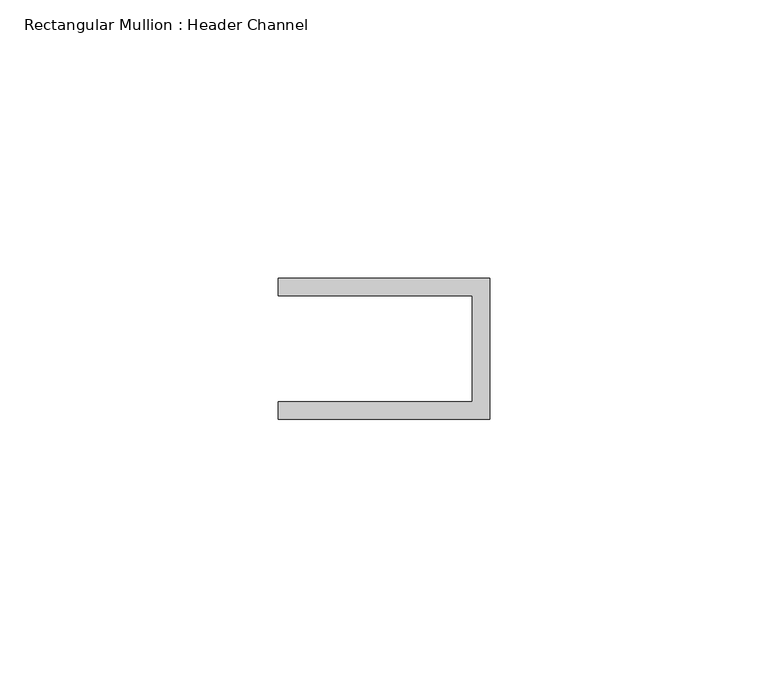
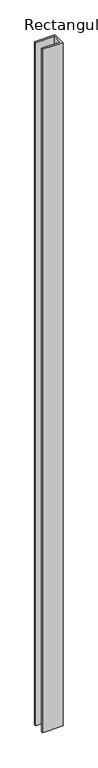
"""IFC4 building model written with IfcOpenShell, lengths in millimetres: member geometry, Rectangular Mullion : Header Channel."""

import ifcopenshell
import ifcopenshell.guid

model = None  # the IFC model being written
_history = None  # IfcOwnerHistory: only IFC2X3 demands one
_inside = {}  # id of a spatial element -> (the spatial element, [elements in it])
_under = {}  # id of a project, library or spatial element -> (it, [spatial elements below it])
_declared = {}  # id of a project -> (the project, [libraries it declares])
_typed = {}  # id of a type object -> (the type object, [elements of that type])
_made_of = {}  # id of a material, layer set ... -> (it, [elements and type objects made of it])


def new_model(schema):
    """Start an empty IFC model of exactly this schema.

    Asked for "IFC4X3", IfcOpenShell would pick the latest addendum, in which some entities
    have other attributes; the version numbers below select the first issue.
    IFC2X3 requires an IfcOwnerHistory on every rooted entity: one is made here for all.
    """
    global model, _history
    if schema == "IFC4X3":
        model = ifcopenshell.file(schema_version=(4, 3, 0, 0))
    else:
        model = ifcopenshell.file(schema=schema)
    _inside.clear()
    _under.clear()
    _declared.clear()
    _typed.clear()
    _made_of.clear()
    _history = None
    if model.schema == "IFC2X3":
        org = make("IfcOrganization", Name="unknown")
        user = make(
            "IfcPersonAndOrganization",
            ThePerson=make("IfcPerson", FamilyName="unknown"),
            TheOrganization=org,
        )
        app = make(
            "IfcApplication",
            ApplicationDeveloper=org,
            Version="unknown",
            ApplicationFullName="unknown",
            ApplicationIdentifier="unknown",
        )
        _history = make(
            "IfcOwnerHistory",
            OwningUser=user,
            OwningApplication=app,
            ChangeAction="ADDED",
            CreationDate=0,
        )
    return model


def make(cls, **values):
    """One entity of the class cls with the attributes given. An attribute that is None is left unset."""
    return model.create_entity(
        cls, **{name: value for name, value in values.items() if value is not None}
    )


def rooted(cls, **values):
    """An entity with a GlobalId (a new one), such as an element, a storey or a relation."""
    return make(cls, GlobalId=ifcopenshell.guid.new(), OwnerHistory=_history, **values)


def si_unit(unit_type, name, prefix=None):
    """IfcSIUnit, for example si_unit("LENGTHUNIT", "METRE", prefix="MILLI")."""
    return make("IfcSIUnit", UnitType=unit_type, Prefix=prefix, Name=name)


def assignment(units):
    """IfcUnitAssignment: the units of a project."""
    return None if units is None else make("IfcUnitAssignment", Units=units)


def point(xyz):
    """IfcCartesianPoint."""
    return None if xyz is None else make("IfcCartesianPoint", Coordinates=xyz)


def direction(xyz):
    """IfcDirection."""
    return None if xyz is None else make("IfcDirection", DirectionRatios=xyz)


def frame(location, z_axis=None, x_axis=None):
    """IfcAxis2Placement3D, a coordinate frame: its origin and axes. An axis left out is left unset."""
    return make(
        "IfcAxis2Placement3D",
        Location=point(location),
        Axis=direction(z_axis),
        RefDirection=direction(x_axis),
    )


def origin():
    """The frame at (0, 0, 0) with its axes left unset."""
    return frame((0.0, 0.0, 0.0))


def place(relative_to, where):
    """IfcLocalPlacement: puts the frame where relative to a parent placement (None: the world)."""
    return make(
        "IfcLocalPlacement", PlacementRelTo=relative_to, RelativePlacement=where
    )


def context(
    kind, dimensions, precision=None, world=None, true_north=None, identifier=None
):
    """IfcGeometricRepresentationContext, for example the 3D "Model" context."""
    return make(
        "IfcGeometricRepresentationContext",
        ContextIdentifier=identifier,
        ContextType=kind,
        CoordinateSpaceDimension=dimensions,
        Precision=precision,
        WorldCoordinateSystem=world,
        TrueNorth=true_north,
    )


def project(units=None, contexts=None):
    """IfcProject with its units and contexts."""
    return rooted(
        "IfcProject",
        Name="project",
        RepresentationContexts=contexts,
        UnitsInContext=assignment(units),
    )


def spatial(cls, under=None, at=None, **own):
    """A site, building, storey or space (cls), placed at a placement, below another one or the project."""
    s = rooted(cls, ObjectPlacement=at, **own)
    if under is not None:
        _under.setdefault(under.id(), (under, []))[1].append(s)
    return s


def polyline(points):
    """IfcPolyline through the points."""
    return make("IfcPolyline", Points=[point(p) for p in points])


def outline(outer, holes=None, kind="AREA"):
    """IfcArbitraryClosedProfileDef: a profile drawn as a closed curve; with holes, ...WithVoids."""
    if holes is None:
        return make("IfcArbitraryClosedProfileDef", ProfileType=kind, OuterCurve=outer)
    return make(
        "IfcArbitraryProfileDefWithVoids",
        ProfileType=kind,
        OuterCurve=outer,
        InnerCurves=holes,
    )


def extrude(swept, where, along, depth):
    """IfcExtrudedAreaSolid: the profile swept, set in the frame where, extruded along a direction by depth."""
    return make(
        "IfcExtrudedAreaSolid",
        SweptArea=swept,
        Position=where,
        ExtrudedDirection=direction(along),
        Depth=depth,
    )


def shape(context_of_items, identifier, shape_type, items):
    """IfcShapeRepresentation: the items that make up one representation, for example the "Body"."""
    return make(
        "IfcShapeRepresentation",
        ContextOfItems=context_of_items,
        RepresentationIdentifier=identifier,
        RepresentationType=shape_type,
        Items=items,
    )


def source(mapping_origin, context_of_items, identifier, shape_type, items):
    """IfcRepresentationMap: a shape defined once, which mapped items show again and again."""
    return make(
        "IfcRepresentationMap",
        MappingOrigin=mapping_origin,
        MappedRepresentation=shape(context_of_items, identifier, shape_type, items),
    )


def transform(
    local_origin,
    x_axis=None,
    y_axis=None,
    z_axis=None,
    scale=None,
    scale2=None,
    scale3=None,
    uniform=True,
):
    """IfcCartesianTransformationOperator3D, or its non-uniform kind. x_axis, y_axis, z_axis: its Axis1, 2, 3."""
    if uniform:
        return make(
            "IfcCartesianTransformationOperator3D",
            Axis1=direction(x_axis),
            Axis2=direction(y_axis),
            LocalOrigin=point(local_origin),
            Scale=scale,
            Axis3=direction(z_axis),
        )
    return make(
        "IfcCartesianTransformationOperator3DnonUniform",
        Axis1=direction(x_axis),
        Axis2=direction(y_axis),
        LocalOrigin=point(local_origin),
        Scale=scale,
        Axis3=direction(z_axis),
        Scale2=scale2,
        Scale3=scale3,
    )


def mapped(mapping_source, mapping_target):
    """IfcMappedItem: shows the shape of a source again, moved by a transform."""
    return make(
        "IfcMappedItem", MappingSource=mapping_source, MappingTarget=mapping_target
    )


def made_of(thing, what):
    """Note that an element or type object is made of a material, layer set ...; save() writes the relation."""
    if what is not None:
        _made_of.setdefault(what.id(), (what, []))[1].append(thing)
    return thing


def element(
    cls,
    number,
    at=None,
    inside=None,
    cuts=None,
    type_object=None,
    material=None,
    context=None,
    identifier="Body",
    shape_type=None,
    held_by="IfcProductDefinitionShape",
    body=None,
    shapes=None,
    **own,
):
    """One element of the class cls, such as IfcWall. Its Tag is "e" and its number.

    at: its placement. inside: the storey or other place that contains it. cuts: it is an
    opening in that element (IfcRelVoidsElement). A single representation is given by context,
    identifier, shape_type and body (its items); several are given by shapes. held_by: the class
    of the entity that holds the representations. save() writes the other relations.
    """
    e = rooted(cls, Tag="e%d" % number, ObjectPlacement=at, **own)
    if body is not None:
        shapes = [shape(context, identifier, shape_type, body)]
    if shapes is not None:
        e.Representation = make(held_by, Representations=shapes)
    if inside is not None:
        _inside.setdefault(inside.id(), (inside, []))[1].append(e)
    if cuts is not None:
        rooted(
            "IfcRelVoidsElement", RelatingBuildingElement=cuts, RelatedOpeningElement=e
        )
    if type_object is not None:
        _typed.setdefault(type_object.id(), (type_object, []))[1].append(e)
    return made_of(e, material)


def aggregate(whole, parts):
    """IfcRelAggregates: a whole, such as a stair, and the parts it consists of."""
    return rooted("IfcRelAggregates", RelatingObject=whole, RelatedObjects=parts)


def save(model, path):
    """Write the relations noted so far, then the file.

    IfcRelAggregates (storeys below a building ...), IfcRelContainedInSpatialStructure (elements
    in a storey), IfcRelDefinesByType, IfcRelAssociatesMaterial and IfcRelDeclares: one each for
    every whole, place, type object, material and project.
    """
    for whole, parts in _under.values():
        aggregate(whole, parts)
    for where, things in _inside.values():
        rooted(
            "IfcRelContainedInSpatialStructure",
            RelatedElements=things,
            RelatingStructure=where,
        )
    for kind, things in _typed.values():
        rooted("IfcRelDefinesByType", RelatedObjects=things, RelatingType=kind)
    for what, things in _made_of.values():
        rooted("IfcRelAssociatesMaterial", RelatedObjects=things, RelatingMaterial=what)
    for by, libraries in _declared.values():
        rooted("IfcRelDeclares", RelatingContext=by, RelatedDefinitions=libraries)
    model.write(path)


def rectangular_mullion_header_channel_fc845e41(model_context):
    return source(origin(), model_context, "Body", "SweptSolid", [
        extrude(outline(polyline([(0.0, 12.7), (0.0, -12.7), (-38.1, -12.7), (-38.1, -9.525), (-3.175, -9.525), (-3.175, 9.525), (-38.1, 9.525), (-38.1, 12.7), (0.0, 12.7)])), frame((0.0, 0.0, -1352.55), z_axis=(0.0, 0.0, 1.0), x_axis=(1.0, 0.0, 0.0)), (0.0, 0.0, 1.0), 1352.55),
    ])


if __name__ == "__main__":
    model = new_model("IFC4")
    model_context = context("Model", 3, world=origin())
    ifc_project = project(units=[si_unit("LENGTHUNIT", "METRE", prefix="MILLI")], contexts=[model_context])
    site = spatial("IfcSite", under=ifc_project)
    building = spatial("IfcBuilding", under=site)
    placement = place(None, origin())
    rectangular_mullion_header_channel_shape = rectangular_mullion_header_channel_fc845e41(model_context)
    element("IfcMember", 1, ObjectType="Rectangular Mullion : Header Channel", at=placement, inside=building, context=model_context, shape_type="MappedRepresentation", body=[
        mapped(rectangular_mullion_header_channel_shape, transform((0.0, 0.0, 0.0), x_axis=(1.0, 0.0, 0.0), y_axis=(0.0, 1.0, 0.0), z_axis=(0.0, 0.0, 1.0))),
    ])
    save(model, "model.ifc")

# Revit data of these elements
# Type "Rectangular Mullion : Header Channel"
#   built-in parameter 1007322 = 0.0833333 (stored number, unit not read)
#   built-in parameter 1007321 = -0.03125 (stored number, unit not read)
#   built-in parameter 1007320 = 0.0416667 (stored number, unit not read)
# Element 1 (IfcMember, "Rectangular Mullion : Header Channel")
#   Materials on its faces: "ALUM"
# Materials
#   "ALUM": class "Generic", colour RGB 157 157 157, transparency 0, Cost = 0
